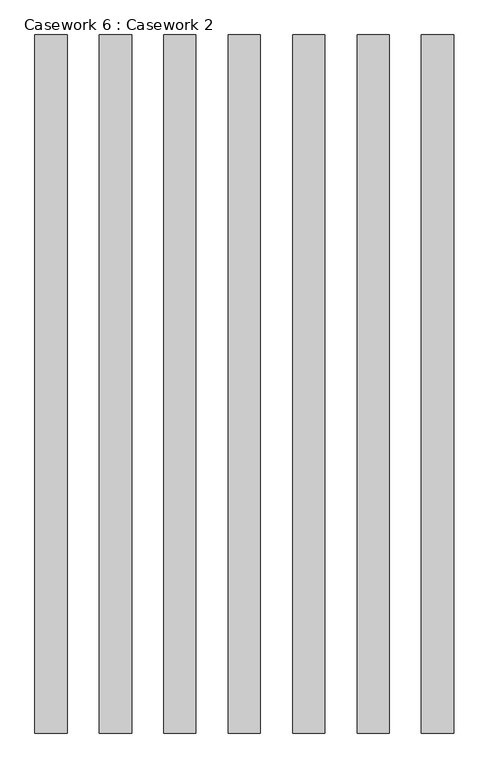
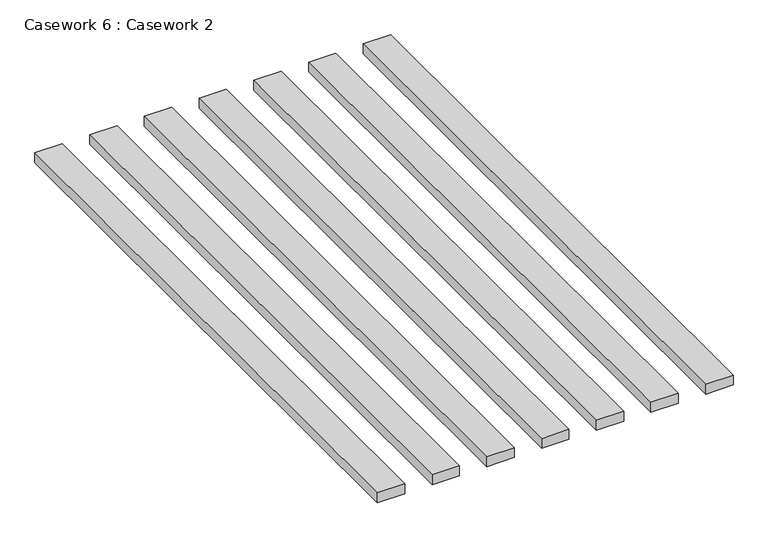
"""IFC4 building model written with IfcOpenShell, lengths in millimetres: furniture geometry, Casework 6 : Casework 2."""

from ifc_helpers import new_model, si_unit, frame, origin, place, context, project, spatial, polyline, outline, extrude, source, transform, mapped, element, save


def casework_6_casework_2_13822944(model_context):
    return source(origin(), model_context, "Body", "SweptSolid", [
        extrude(outline(polyline([(-4948.5247381, 2870.3649316), (-4898.5247381, 2870.3649316), (-4898.5247381, 1786.6149316), (-4948.5247381, 1786.6149316), (-4948.5247381, 2870.3649316)])), frame((0.0, 0.0, 4033.1977901), z_axis=(0.0, 0.0, 1.0), x_axis=(1.0, 0.0, 0.0)), (0.0, 0.0, 1.0), 19.0),
        extrude(outline(polyline([(-4848.5247381, 2870.3649316), (-4798.5247381, 2870.3649316), (-4798.5247381, 1786.6149316), (-4848.5247381, 1786.6149316), (-4848.5247381, 2870.3649316)])), frame((0.0, 0.0, 4033.1977901), z_axis=(0.0, 0.0, 1.0), x_axis=(1.0, 0.0, 0.0)), (0.0, 0.0, 1.0), 19.0),
        extrude(outline(polyline([(-4748.5247381, 2870.3649316), (-4698.5247381, 2870.3649316), (-4698.5247381, 1786.6149316), (-4748.5247381, 1786.6149316), (-4748.5247381, 2870.3649316)])), frame((0.0, 0.0, 4033.1977901), z_axis=(0.0, 0.0, 1.0), x_axis=(1.0, 0.0, 0.0)), (0.0, 0.0, 1.0), 19.0),
        extrude(outline(polyline([(-4648.5247381, 2870.3649316), (-4598.5247381, 2870.3649316), (-4598.5247381, 1786.6149316), (-4648.5247381, 1786.6149316), (-4648.5247381, 2870.3649316)])), frame((0.0, 0.0, 4033.1977901), z_axis=(0.0, 0.0, 1.0), x_axis=(1.0, 0.0, 0.0)), (0.0, 0.0, 1.0), 19.0),
        extrude(outline(polyline([(-4548.5247381, 2870.3649316), (-4498.5247381, 2870.3649316), (-4498.5247381, 1786.6149316), (-4548.5247381, 1786.6149316), (-4548.5247381, 2870.3649316)])), frame((0.0, 0.0, 4033.1977901), z_axis=(0.0, 0.0, 1.0), x_axis=(1.0, 0.0, 0.0)), (0.0, 0.0, 1.0), 19.0),
        extrude(outline(polyline([(-4448.5247381, 2870.3649316), (-4398.5247381, 2870.3649316), (-4398.5247381, 1786.6149316), (-4448.5247381, 1786.6149316), (-4448.5247381, 2870.3649316)])), frame((0.0, 0.0, 4033.1977901), z_axis=(0.0, 0.0, 1.0), x_axis=(1.0, 0.0, 0.0)), (0.0, 0.0, 1.0), 19.0),
        extrude(outline(polyline([(-4348.5247381, 2870.3649316), (-4298.5247381, 2870.3649316), (-4298.5247381, 1786.6149316), (-4348.5247381, 1786.6149316), (-4348.5247381, 2870.3649316)])), frame((0.0, 0.0, 4033.1977901), z_axis=(0.0, 0.0, 1.0), x_axis=(1.0, 0.0, 0.0)), (0.0, 0.0, 1.0), 19.0),
    ])


if __name__ == "__main__":
    model = new_model("IFC4")
    model_context = context("Model", 3, world=origin())
    ifc_project = project(units=[si_unit("LENGTHUNIT", "METRE", prefix="MILLI")], contexts=[model_context])
    site = spatial("IfcSite", under=ifc_project)
    building = spatial("IfcBuilding", under=site)
    placement = place(None, origin())
    casework_6_casework_2_shape = casework_6_casework_2_13822944(model_context)
    element("IfcFurniture", 1, ObjectType="Casework 6 : Casework 2", at=placement, inside=building, context=model_context, shape_type="MappedRepresentation", body=[
        mapped(casework_6_casework_2_shape, transform((0.0, 0.0, 0.0), x_axis=(1.0, 0.0, 0.0), y_axis=(0.0, 1.0, 0.0), z_axis=(0.0, 0.0, 1.0))),
    ])
    save(model, "model.ifc")
